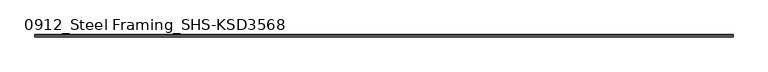
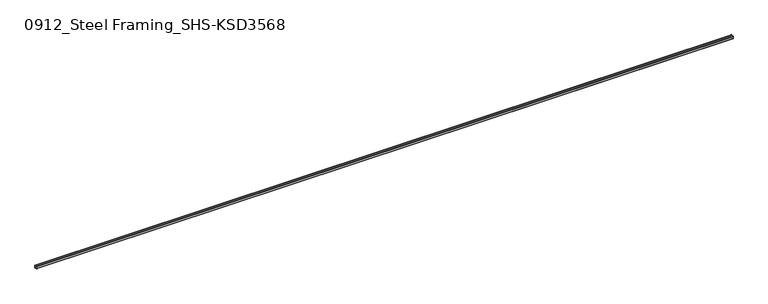
"""IFC4 building model written with IfcOpenShell, lengths in millimetres: beam geometry, 0912_Steel Framing_SHS-KSD3568 : H_SB_ASB_SHS-150x150x6."""

import ifcopenshell
import ifcopenshell.guid

model = None  # the IFC model being written
_history = None  # IfcOwnerHistory: only IFC2X3 demands one
_inside = {}  # id of a spatial element -> (the spatial element, [elements in it])
_under = {}  # id of a project, library or spatial element -> (it, [spatial elements below it])
_declared = {}  # id of a project -> (the project, [libraries it declares])
_typed = {}  # id of a type object -> (the type object, [elements of that type])
_made_of = {}  # id of a material, layer set ... -> (it, [elements and type objects made of it])


def new_model(schema):
    """Start an empty IFC model of exactly this schema.

    Asked for "IFC4X3", IfcOpenShell would pick the latest addendum, in which some entities
    have other attributes; the version numbers below select the first issue.
    IFC2X3 requires an IfcOwnerHistory on every rooted entity: one is made here for all.
    """
    global model, _history
    if schema == "IFC4X3":
        model = ifcopenshell.file(schema_version=(4, 3, 0, 0))
    else:
        model = ifcopenshell.file(schema=schema)
    _inside.clear()
    _under.clear()
    _declared.clear()
    _typed.clear()
    _made_of.clear()
    _history = None
    if model.schema == "IFC2X3":
        org = make("IfcOrganization", Name="unknown")
        user = make(
            "IfcPersonAndOrganization",
            ThePerson=make("IfcPerson", FamilyName="unknown"),
            TheOrganization=org,
        )
        app = make(
            "IfcApplication",
            ApplicationDeveloper=org,
            Version="unknown",
            ApplicationFullName="unknown",
            ApplicationIdentifier="unknown",
        )
        _history = make(
            "IfcOwnerHistory",
            OwningUser=user,
            OwningApplication=app,
            ChangeAction="ADDED",
            CreationDate=0,
        )
    return model


def make(cls, **values):
    """One entity of the class cls with the attributes given. An attribute that is None is left unset."""
    return model.create_entity(
        cls, **{name: value for name, value in values.items() if value is not None}
    )


def rooted(cls, **values):
    """An entity with a GlobalId (a new one), such as an element, a storey or a relation."""
    return make(cls, GlobalId=ifcopenshell.guid.new(), OwnerHistory=_history, **values)


def si_unit(unit_type, name, prefix=None):
    """IfcSIUnit, for example si_unit("LENGTHUNIT", "METRE", prefix="MILLI")."""
    return make("IfcSIUnit", UnitType=unit_type, Prefix=prefix, Name=name)


def assignment(units):
    """IfcUnitAssignment: the units of a project."""
    return None if units is None else make("IfcUnitAssignment", Units=units)


def point(xyz):
    """IfcCartesianPoint."""
    return None if xyz is None else make("IfcCartesianPoint", Coordinates=xyz)


def direction(xyz):
    """IfcDirection."""
    return None if xyz is None else make("IfcDirection", DirectionRatios=xyz)


def frame(location, z_axis=None, x_axis=None):
    """IfcAxis2Placement3D, a coordinate frame: its origin and axes. An axis left out is left unset."""
    return make(
        "IfcAxis2Placement3D",
        Location=point(location),
        Axis=direction(z_axis),
        RefDirection=direction(x_axis),
    )


def frame_2d(location, x_axis=None):
    """IfcAxis2Placement2D, a coordinate frame in the plane: its origin and x axis."""
    return make(
        "IfcAxis2Placement2D", Location=point(location), RefDirection=direction(x_axis)
    )


def origin():
    """The frame at (0, 0, 0) with its axes left unset."""
    return frame((0.0, 0.0, 0.0))


def place(relative_to, where):
    """IfcLocalPlacement: puts the frame where relative to a parent placement (None: the world)."""
    return make(
        "IfcLocalPlacement", PlacementRelTo=relative_to, RelativePlacement=where
    )


def context(
    kind, dimensions, precision=None, world=None, true_north=None, identifier=None
):
    """IfcGeometricRepresentationContext, for example the 3D "Model" context."""
    return make(
        "IfcGeometricRepresentationContext",
        ContextIdentifier=identifier,
        ContextType=kind,
        CoordinateSpaceDimension=dimensions,
        Precision=precision,
        WorldCoordinateSystem=world,
        TrueNorth=true_north,
    )


def project(units=None, contexts=None):
    """IfcProject with its units and contexts."""
    return rooted(
        "IfcProject",
        Name="project",
        RepresentationContexts=contexts,
        UnitsInContext=assignment(units),
    )


def spatial(cls, under=None, at=None, **own):
    """A site, building, storey or space (cls), placed at a placement, below another one or the project."""
    s = rooted(cls, ObjectPlacement=at, **own)
    if under is not None:
        _under.setdefault(under.id(), (under, []))[1].append(s)
    return s


def polyline(points):
    """IfcPolyline through the points."""
    return make("IfcPolyline", Points=[point(p) for p in points])


def circle_curve(where, radius):
    """IfcCircle in the frame where."""
    return make("IfcCircle", Position=where, Radius=radius)


def trimmed(basis, trim1, trim2, sense, master):
    """IfcTrimmedCurve: the piece of a basis curve between two trims."""
    return make(
        "IfcTrimmedCurve",
        BasisCurve=basis,
        Trim1=trim1,
        Trim2=trim2,
        SenseAgreement=sense,
        MasterRepresentation=master,
    )


def segment(curve, same_sense, transition):
    """IfcCompositeCurveSegment."""
    return make(
        "IfcCompositeCurveSegment",
        Transition=transition,
        SameSense=same_sense,
        ParentCurve=curve,
    )


def composite_curve(segments, self_intersect=None):
    """IfcCompositeCurve: segments joined end to end."""
    return make("IfcCompositeCurve", Segments=segments, SelfIntersect=self_intersect)


def outline(outer, holes=None, kind="AREA"):
    """IfcArbitraryClosedProfileDef: a profile drawn as a closed curve; with holes, ...WithVoids."""
    if holes is None:
        return make("IfcArbitraryClosedProfileDef", ProfileType=kind, OuterCurve=outer)
    return make(
        "IfcArbitraryProfileDefWithVoids",
        ProfileType=kind,
        OuterCurve=outer,
        InnerCurves=holes,
    )


def extrude(swept, where, along, depth):
    """IfcExtrudedAreaSolid: the profile swept, set in the frame where, extruded along a direction by depth."""
    return make(
        "IfcExtrudedAreaSolid",
        SweptArea=swept,
        Position=where,
        ExtrudedDirection=direction(along),
        Depth=depth,
    )


def shape(context_of_items, identifier, shape_type, items):
    """IfcShapeRepresentation: the items that make up one representation, for example the "Body"."""
    return make(
        "IfcShapeRepresentation",
        ContextOfItems=context_of_items,
        RepresentationIdentifier=identifier,
        RepresentationType=shape_type,
        Items=items,
    )


def source(mapping_origin, context_of_items, identifier, shape_type, items):
    """IfcRepresentationMap: a shape defined once, which mapped items show again and again."""
    return make(
        "IfcRepresentationMap",
        MappingOrigin=mapping_origin,
        MappedRepresentation=shape(context_of_items, identifier, shape_type, items),
    )


def transform(
    local_origin,
    x_axis=None,
    y_axis=None,
    z_axis=None,
    scale=None,
    scale2=None,
    scale3=None,
    uniform=True,
):
    """IfcCartesianTransformationOperator3D, or its non-uniform kind. x_axis, y_axis, z_axis: its Axis1, 2, 3."""
    if uniform:
        return make(
            "IfcCartesianTransformationOperator3D",
            Axis1=direction(x_axis),
            Axis2=direction(y_axis),
            LocalOrigin=point(local_origin),
            Scale=scale,
            Axis3=direction(z_axis),
        )
    return make(
        "IfcCartesianTransformationOperator3DnonUniform",
        Axis1=direction(x_axis),
        Axis2=direction(y_axis),
        LocalOrigin=point(local_origin),
        Scale=scale,
        Axis3=direction(z_axis),
        Scale2=scale2,
        Scale3=scale3,
    )


def mapped(mapping_source, mapping_target):
    """IfcMappedItem: shows the shape of a source again, moved by a transform."""
    return make(
        "IfcMappedItem", MappingSource=mapping_source, MappingTarget=mapping_target
    )


def made_of(thing, what):
    """Note that an element or type object is made of a material, layer set ...; save() writes the relation."""
    if what is not None:
        _made_of.setdefault(what.id(), (what, []))[1].append(thing)
    return thing


def element(
    cls,
    number,
    at=None,
    inside=None,
    cuts=None,
    type_object=None,
    material=None,
    context=None,
    identifier="Body",
    shape_type=None,
    held_by="IfcProductDefinitionShape",
    body=None,
    shapes=None,
    **own,
):
    """One element of the class cls, such as IfcWall. Its Tag is "e" and its number.

    at: its placement. inside: the storey or other place that contains it. cuts: it is an
    opening in that element (IfcRelVoidsElement). A single representation is given by context,
    identifier, shape_type and body (its items); several are given by shapes. held_by: the class
    of the entity that holds the representations. save() writes the other relations.
    """
    e = rooted(cls, Tag="e%d" % number, ObjectPlacement=at, **own)
    if body is not None:
        shapes = [shape(context, identifier, shape_type, body)]
    if shapes is not None:
        e.Representation = make(held_by, Representations=shapes)
    if inside is not None:
        _inside.setdefault(inside.id(), (inside, []))[1].append(e)
    if cuts is not None:
        rooted(
            "IfcRelVoidsElement", RelatingBuildingElement=cuts, RelatedOpeningElement=e
        )
    if type_object is not None:
        _typed.setdefault(type_object.id(), (type_object, []))[1].append(e)
    return made_of(e, material)


def aggregate(whole, parts):
    """IfcRelAggregates: a whole, such as a stair, and the parts it consists of."""
    return rooted("IfcRelAggregates", RelatingObject=whole, RelatedObjects=parts)


def save(model, path):
    """Write the relations noted so far, then the file.

    IfcRelAggregates (storeys below a building ...), IfcRelContainedInSpatialStructure (elements
    in a storey), IfcRelDefinesByType, IfcRelAssociatesMaterial and IfcRelDeclares: one each for
    every whole, place, type object, material and project.
    """
    for whole, parts in _under.values():
        aggregate(whole, parts)
    for where, things in _inside.values():
        rooted(
            "IfcRelContainedInSpatialStructure",
            RelatedElements=things,
            RelatingStructure=where,
        )
    for kind, things in _typed.values():
        rooted("IfcRelDefinesByType", RelatedObjects=things, RelatingType=kind)
    for what, things in _made_of.values():
        rooted("IfcRelAssociatesMaterial", RelatedObjects=things, RelatingMaterial=what)
    for by, libraries in _declared.values():
        rooted("IfcRelDeclares", RelatingContext=by, RelatedDefinitions=libraries)
    model.write(path)


def beam_0912_steel_framing_shs_ksd3568_c1333ee6(model_context):
    return source(origin(), model_context, "Body", "SweptSolid", [
        extrude(outline(composite_curve([segment(polyline([(75.0, 63.0), (75.0, -63.0)]), True, "CONTINUOUS"), segment(trimmed(circle_curve(frame_2d((63.0, -63.0)), 12.0), [point((75.0, -63.0))], [point((63.0, -75.0))], False, "CARTESIAN"), True, "CONTINUOUS"), segment(polyline([(63.0, -75.0), (-63.0, -75.0)]), True, "CONTINUOUS"), segment(trimmed(circle_curve(frame_2d((-63.0, -63.0)), 12.0), [point((-63.0, -75.0))], [point((-75.0, -63.0))], False, "CARTESIAN"), True, "CONTINUOUS"), segment(polyline([(-75.0, -63.0), (-75.0, 63.0)]), True, "CONTINUOUS"), segment(trimmed(circle_curve(frame_2d((-63.0, 63.0)), 12.0), [point((-75.0, 63.0))], [point((-63.0, 75.0))], False, "CARTESIAN"), True, "CONTINUOUS"), segment(polyline([(-63.0, 75.0), (63.0, 75.0)]), True, "CONTINUOUS"), segment(trimmed(circle_curve(frame_2d((63.0, 63.0)), 12.0), [point((63.0, 75.0))], [point((75.0, 63.0))], False, "CARTESIAN"), True, "CONTINUOUS")], self_intersect=False), holes=[composite_curve([segment(trimmed(circle_curve(frame_2d((-63.0, 63.0)), 6.0), [point((-63.0, 69.0))], [point((-69.0, 63.0))], True, "CARTESIAN"), True, "CONTINUOUS"), segment(polyline([(-69.0, 63.0), (-69.0, -63.0)]), True, "CONTINUOUS"), segment(trimmed(circle_curve(frame_2d((-63.0, -63.0)), 6.0), [point((-69.0, -63.0))], [point((-63.0, -69.0))], True, "CARTESIAN"), True, "CONTINUOUS"), segment(polyline([(-63.0, -69.0), (63.0, -69.0)]), True, "CONTINUOUS"), segment(trimmed(circle_curve(frame_2d((63.0, -63.0)), 6.0), [point((63.0, -69.0))], [point((69.0, -63.0))], True, "CARTESIAN"), True, "CONTINUOUS"), segment(polyline([(69.0, -63.0), (69.0, 63.0)]), True, "CONTINUOUS"), segment(trimmed(circle_curve(frame_2d((63.0, 63.0)), 6.0), [point((69.0, 63.0))], [point((63.0, 69.0))], True, "CARTESIAN"), True, "CONTINUOUS"), segment(polyline([(63.0, 69.0), (-63.0, 69.0)]), True, "CONTINUOUS")], self_intersect=False)]), frame((-20547.5, 0.0, 0.0), z_axis=(1.0, 0.0, 0.0), x_axis=(0.0, 1.0, 0.0)), (0.0, 0.0, 1.0), 41095.0),
    ])


if __name__ == "__main__":
    model = new_model("IFC4")
    model_context = context("Model", 3, world=origin())
    ifc_project = project(units=[si_unit("LENGTHUNIT", "METRE", prefix="MILLI")], contexts=[model_context])
    site = spatial("IfcSite", under=ifc_project)
    building = spatial("IfcBuilding", under=site)
    placement = place(None, origin())
    beam_0912_steel_framing_shs_ksd3568_shape = beam_0912_steel_framing_shs_ksd3568_c1333ee6(model_context)
    element("IfcBeam", 1, ObjectType="0912_Steel Framing_SHS-KSD3568 : H_SB_ASB_SHS-150x150x6", at=placement, inside=building, context=model_context, shape_type="MappedRepresentation", body=[
        mapped(beam_0912_steel_framing_shs_ksd3568_shape, transform((0.0, 0.0, 0.0), x_axis=(1.0, 0.0, 0.0), y_axis=(0.0, 1.0, 0.0), z_axis=(0.0, 0.0, 1.0))),
    ])
    save(model, "model.ifc")

# Revit data of these elements
# Type "0912_Steel Framing_SHS-KSD3568 : H_SB_ASB_SHS-150x150x6"
#   H_WM Code_1 = "S01AA002-00001 | Main Steel Structure Fabrication Work | Shelter/Building | Medium Steel - Standard (90KG/M>Weight≥30KG/M) | Material: (   )"
#   H_WM Code_2 = "S03AA028-00001 | Main Steel Structure Erection Work | Shelter/Building | Medium Steel (90KG/M>Weight≥30KG/M) | Material: (   )"
#   H_WM Code_3 = "S01AA010-00001 | Main Steel Structure Fabrication Work | Shelter/Building | Steel Painting/Coating | for Non-Fireproofed Steel Surface, Surface Preparation, Primer, Second & Final Coat | Material: (   )"
#   H_Q'ty Cal Type Tag = "SB-Q2"
#   Perimeter = 0.60 m²/m
#   Nominal Weight = 26.40 kgf/m
#   Length [instance default] = 1.0000 m
#   b = 0.1500 m
#   h = 0.1500 m
#   tr = 0.0120 m
#   t = 0.0060 m
#   A = 28.36 m²
#   Structural Material [instance default] = Steel, 45-345
# Element 1 (IfcBeam, "0912_Steel Framing_SHS-KSD3568 : H_SB_ASB_SHS-150x150x6")
#   Structural Material = none
# Materials
#   "Steel, 45-345": class "Metal", colour RGB 189 187 185, transparency 0, Description = "Steel 345 MPa", Cost = 0
